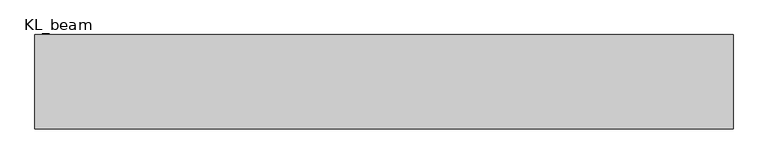
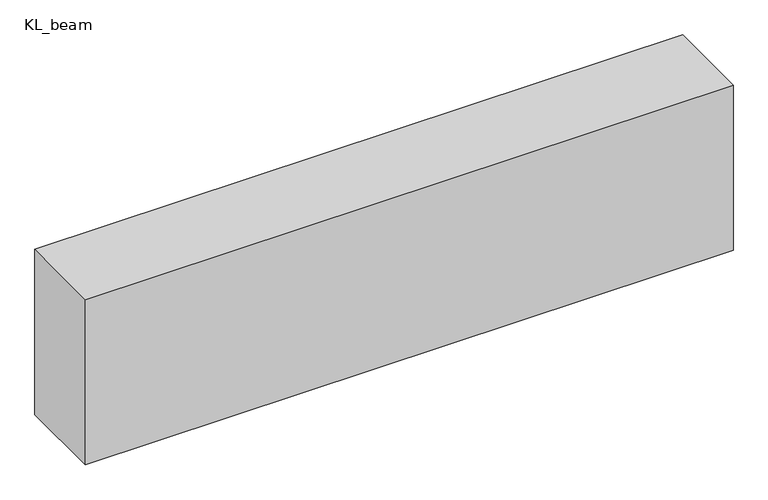
"""IFC4 building model written with IfcOpenShell, lengths in millimetres: beam geometry, 混凝土 - 矩形梁 : KL_beam."""

from ifc_helpers import new_model, si_unit, frame, origin, place, context, project, spatial, polyline, outline, extrude, source, transform, mapped, element, save


def kl_beam_28a16925(model_context):
    return source(origin(), model_context, "Body", "SweptSolid", [
        extrude(outline(polyline([(1483.0, 200.0), (1483.0, -200.0), (-1483.0, -200.0), (-1483.0, 200.0), (1483.0, 200.0)])), frame((0.0, 0.0, -400.0), z_axis=(0.0, 0.0, 1.0), x_axis=(1.0, 0.0, 0.0)), (0.0, 0.0, 1.0), 800.0),
    ])


if __name__ == "__main__":
    model = new_model("IFC4")
    model_context = context("Model", 3, world=origin())
    ifc_project = project(units=[si_unit("LENGTHUNIT", "METRE", prefix="MILLI")], contexts=[model_context])
    site = spatial("IfcSite", under=ifc_project)
    building = spatial("IfcBuilding", under=site)
    placement = place(None, origin())
    kl_beam_shape = kl_beam_28a16925(model_context)
    element("IfcBeam", 1, ObjectType="混凝土 - 矩形梁 : KL_beam", at=placement, inside=building, context=model_context, shape_type="MappedRepresentation", body=[
        mapped(kl_beam_shape, transform((0.0, 0.0, 0.0), x_axis=(1.0, 0.0, 0.0), y_axis=(0.0, 1.0, 0.0), z_axis=(0.0, 0.0, 1.0))),
    ])
    save(model, "model.ifc")

# Revit data of these elements
# Type "混凝土 - 矩形梁 : KL_beam"
#   Length [instance default] = 1524 mm
#   b = 400 mm
#   h = 800 mm
#   Structural Material [instance default] = 混凝土 - 现场浇注混凝土
#   Assembly Code = ""
# Element 1 (IfcBeam, "混凝土 - 矩形梁 : KL_beam")
#   Structural Material = none
# Materials
#   "混凝土 - 现场浇注混凝土": class "混凝土", colour RGB 192 192 192, transparency 0
